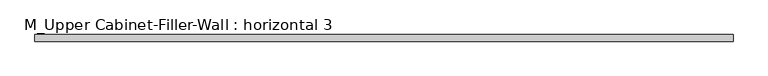
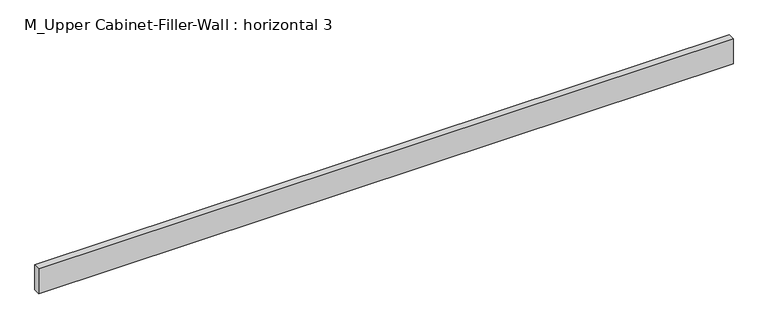
"""IFC4 building model written with IfcOpenShell, lengths in millimetres: furniture geometry, M_Upper Cabinet-Filler-Wall : horizontal 3."""

from ifc_helpers import new_model, si_unit, frame, origin, place, context, project, spatial, polyline, outline, extrude, source, transform, mapped, element, save


def m_upper_cabinet_filler_wall_horizontal_3_602a78bd(model_context):
    return source(origin(), model_context, "Body", "SweptSolid", [
        extrude(outline(polyline([(-967.1788372, 38.1), (-967.1788372, 57.15), (1026.7211628, 57.15), (1026.7211628, 38.1), (-967.1788372, 38.1)])), frame((0.0, 0.0, 1923.8), z_axis=(0.0, 0.0, 1.0), x_axis=(1.0, 0.0, 0.0)), (0.0, 0.0, 1.0), 76.2),
    ])


if __name__ == "__main__":
    model = new_model("IFC4")
    model_context = context("Model", 3, world=origin())
    ifc_project = project(units=[si_unit("LENGTHUNIT", "METRE", prefix="MILLI")], contexts=[model_context])
    site = spatial("IfcSite", under=ifc_project)
    building = spatial("IfcBuilding", under=site)
    placement = place(None, origin())
    m_upper_cabinet_filler_wall_horizontal_3_shape = m_upper_cabinet_filler_wall_horizontal_3_602a78bd(model_context)
    element("IfcFurniture", 1, ObjectType="M_Upper Cabinet-Filler-Wall : horizontal 3", at=placement, inside=building, context=model_context, shape_type="MappedRepresentation", body=[
        mapped(m_upper_cabinet_filler_wall_horizontal_3_shape, transform((0.0, 0.0, 0.0), x_axis=(1.0, 0.0, 0.0), y_axis=(0.0, 1.0, 0.0), z_axis=(0.0, 0.0, 1.0))),
    ])
    save(model, "model.ifc")

# Revit data of these elements
# Type "M_Upper Cabinet-Filler-Wall : horizontal 3"
#   Depth = 0' - 1"
#   Height = 0' - 3"
#   Top Of Cabinet = 6' - 6.74016"
#   Width = 6' - 6 1/2"
#   Cabinet Material = none
#   Default Elevation = 0
# Element 1 (IfcFurniture, "M_Upper Cabinet-Filler-Wall : horizontal 3")
#   Materials on its faces: "Cabinets"
# Materials
#   "Cabinets": class "Miscellaneous", colour RGB 249 249 249, transparency 0
